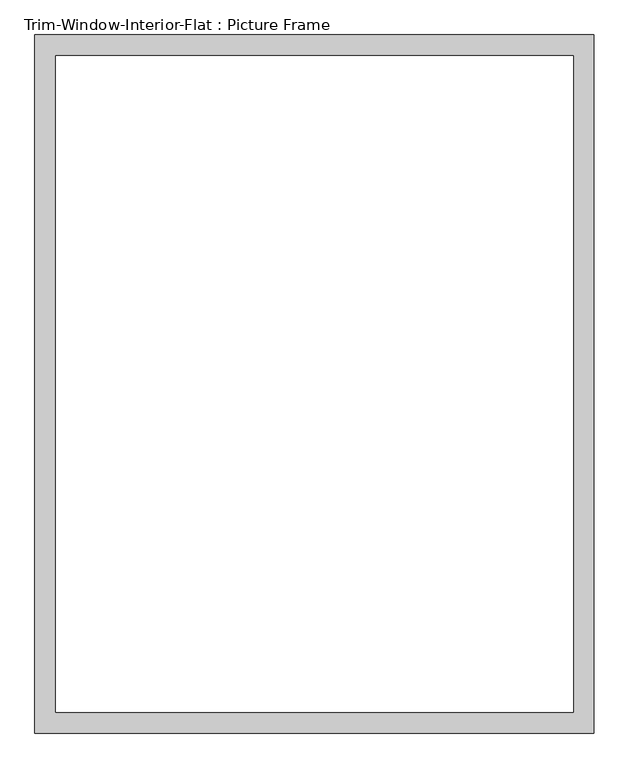
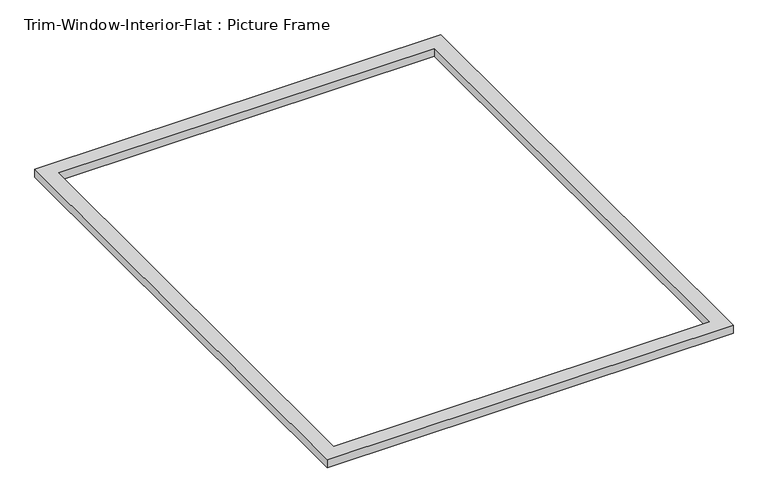
"""IFC4 building model written with IfcOpenShell, lengths in millimetres: proxy geometry, Trim-Window-Interior-Flat : Picture Frame."""

import ifcopenshell
import ifcopenshell.guid

model = None  # the IFC model being written
_history = None  # IfcOwnerHistory: only IFC2X3 demands one
_inside = {}  # id of a spatial element -> (the spatial element, [elements in it])
_under = {}  # id of a project, library or spatial element -> (it, [spatial elements below it])
_declared = {}  # id of a project -> (the project, [libraries it declares])
_typed = {}  # id of a type object -> (the type object, [elements of that type])
_made_of = {}  # id of a material, layer set ... -> (it, [elements and type objects made of it])


def new_model(schema):
    """Start an empty IFC model of exactly this schema.

    Asked for "IFC4X3", IfcOpenShell would pick the latest addendum, in which some entities
    have other attributes; the version numbers below select the first issue.
    IFC2X3 requires an IfcOwnerHistory on every rooted entity: one is made here for all.
    """
    global model, _history
    if schema == "IFC4X3":
        model = ifcopenshell.file(schema_version=(4, 3, 0, 0))
    else:
        model = ifcopenshell.file(schema=schema)
    _inside.clear()
    _under.clear()
    _declared.clear()
    _typed.clear()
    _made_of.clear()
    _history = None
    if model.schema == "IFC2X3":
        org = make("IfcOrganization", Name="unknown")
        user = make(
            "IfcPersonAndOrganization",
            ThePerson=make("IfcPerson", FamilyName="unknown"),
            TheOrganization=org,
        )
        app = make(
            "IfcApplication",
            ApplicationDeveloper=org,
            Version="unknown",
            ApplicationFullName="unknown",
            ApplicationIdentifier="unknown",
        )
        _history = make(
            "IfcOwnerHistory",
            OwningUser=user,
            OwningApplication=app,
            ChangeAction="ADDED",
            CreationDate=0,
        )
    return model


def make(cls, **values):
    """One entity of the class cls with the attributes given. An attribute that is None is left unset."""
    return model.create_entity(
        cls, **{name: value for name, value in values.items() if value is not None}
    )


def rooted(cls, **values):
    """An entity with a GlobalId (a new one), such as an element, a storey or a relation."""
    return make(cls, GlobalId=ifcopenshell.guid.new(), OwnerHistory=_history, **values)


def si_unit(unit_type, name, prefix=None):
    """IfcSIUnit, for example si_unit("LENGTHUNIT", "METRE", prefix="MILLI")."""
    return make("IfcSIUnit", UnitType=unit_type, Prefix=prefix, Name=name)


def assignment(units):
    """IfcUnitAssignment: the units of a project."""
    return None if units is None else make("IfcUnitAssignment", Units=units)


def point(xyz):
    """IfcCartesianPoint."""
    return None if xyz is None else make("IfcCartesianPoint", Coordinates=xyz)


def direction(xyz):
    """IfcDirection."""
    return None if xyz is None else make("IfcDirection", DirectionRatios=xyz)


def frame(location, z_axis=None, x_axis=None):
    """IfcAxis2Placement3D, a coordinate frame: its origin and axes. An axis left out is left unset."""
    return make(
        "IfcAxis2Placement3D",
        Location=point(location),
        Axis=direction(z_axis),
        RefDirection=direction(x_axis),
    )


def origin():
    """The frame at (0, 0, 0) with its axes left unset."""
    return frame((0.0, 0.0, 0.0))


def origin_with_axes():
    """The frame at (0, 0, 0) with the z axis (0, 0, 1) and the x axis (1, 0, 0) written out."""
    return frame((0.0, 0.0, 0.0), z_axis=(0.0, 0.0, 1.0), x_axis=(1.0, 0.0, 0.0))


def place(relative_to, where):
    """IfcLocalPlacement: puts the frame where relative to a parent placement (None: the world)."""
    return make(
        "IfcLocalPlacement", PlacementRelTo=relative_to, RelativePlacement=where
    )


def context(
    kind, dimensions, precision=None, world=None, true_north=None, identifier=None
):
    """IfcGeometricRepresentationContext, for example the 3D "Model" context."""
    return make(
        "IfcGeometricRepresentationContext",
        ContextIdentifier=identifier,
        ContextType=kind,
        CoordinateSpaceDimension=dimensions,
        Precision=precision,
        WorldCoordinateSystem=world,
        TrueNorth=true_north,
    )


def project(units=None, contexts=None):
    """IfcProject with its units and contexts."""
    return rooted(
        "IfcProject",
        Name="project",
        RepresentationContexts=contexts,
        UnitsInContext=assignment(units),
    )


def spatial(cls, under=None, at=None, **own):
    """A site, building, storey or space (cls), placed at a placement, below another one or the project."""
    s = rooted(cls, ObjectPlacement=at, **own)
    if under is not None:
        _under.setdefault(under.id(), (under, []))[1].append(s)
    return s


def polyline(points):
    """IfcPolyline through the points."""
    return make("IfcPolyline", Points=[point(p) for p in points])


def outline(outer, holes=None, kind="AREA"):
    """IfcArbitraryClosedProfileDef: a profile drawn as a closed curve; with holes, ...WithVoids."""
    if holes is None:
        return make("IfcArbitraryClosedProfileDef", ProfileType=kind, OuterCurve=outer)
    return make(
        "IfcArbitraryProfileDefWithVoids",
        ProfileType=kind,
        OuterCurve=outer,
        InnerCurves=holes,
    )


def extrude(swept, where, along, depth):
    """IfcExtrudedAreaSolid: the profile swept, set in the frame where, extruded along a direction by depth."""
    return make(
        "IfcExtrudedAreaSolid",
        SweptArea=swept,
        Position=where,
        ExtrudedDirection=direction(along),
        Depth=depth,
    )


def shape(context_of_items, identifier, shape_type, items):
    """IfcShapeRepresentation: the items that make up one representation, for example the "Body"."""
    return make(
        "IfcShapeRepresentation",
        ContextOfItems=context_of_items,
        RepresentationIdentifier=identifier,
        RepresentationType=shape_type,
        Items=items,
    )


def source(mapping_origin, context_of_items, identifier, shape_type, items):
    """IfcRepresentationMap: a shape defined once, which mapped items show again and again."""
    return make(
        "IfcRepresentationMap",
        MappingOrigin=mapping_origin,
        MappedRepresentation=shape(context_of_items, identifier, shape_type, items),
    )


def transform(
    local_origin,
    x_axis=None,
    y_axis=None,
    z_axis=None,
    scale=None,
    scale2=None,
    scale3=None,
    uniform=True,
):
    """IfcCartesianTransformationOperator3D, or its non-uniform kind. x_axis, y_axis, z_axis: its Axis1, 2, 3."""
    if uniform:
        return make(
            "IfcCartesianTransformationOperator3D",
            Axis1=direction(x_axis),
            Axis2=direction(y_axis),
            LocalOrigin=point(local_origin),
            Scale=scale,
            Axis3=direction(z_axis),
        )
    return make(
        "IfcCartesianTransformationOperator3DnonUniform",
        Axis1=direction(x_axis),
        Axis2=direction(y_axis),
        LocalOrigin=point(local_origin),
        Scale=scale,
        Axis3=direction(z_axis),
        Scale2=scale2,
        Scale3=scale3,
    )


def mapped(mapping_source, mapping_target):
    """IfcMappedItem: shows the shape of a source again, moved by a transform."""
    return make(
        "IfcMappedItem", MappingSource=mapping_source, MappingTarget=mapping_target
    )


def made_of(thing, what):
    """Note that an element or type object is made of a material, layer set ...; save() writes the relation."""
    if what is not None:
        _made_of.setdefault(what.id(), (what, []))[1].append(thing)
    return thing


def element(
    cls,
    number,
    at=None,
    inside=None,
    cuts=None,
    type_object=None,
    material=None,
    context=None,
    identifier="Body",
    shape_type=None,
    held_by="IfcProductDefinitionShape",
    body=None,
    shapes=None,
    **own,
):
    """One element of the class cls, such as IfcWall. Its Tag is "e" and its number.

    at: its placement. inside: the storey or other place that contains it. cuts: it is an
    opening in that element (IfcRelVoidsElement). A single representation is given by context,
    identifier, shape_type and body (its items); several are given by shapes. held_by: the class
    of the entity that holds the representations. save() writes the other relations.
    """
    e = rooted(cls, Tag="e%d" % number, ObjectPlacement=at, **own)
    if body is not None:
        shapes = [shape(context, identifier, shape_type, body)]
    if shapes is not None:
        e.Representation = make(held_by, Representations=shapes)
    if inside is not None:
        _inside.setdefault(inside.id(), (inside, []))[1].append(e)
    if cuts is not None:
        rooted(
            "IfcRelVoidsElement", RelatingBuildingElement=cuts, RelatedOpeningElement=e
        )
    if type_object is not None:
        _typed.setdefault(type_object.id(), (type_object, []))[1].append(e)
    return made_of(e, material)


def aggregate(whole, parts):
    """IfcRelAggregates: a whole, such as a stair, and the parts it consists of."""
    return rooted("IfcRelAggregates", RelatingObject=whole, RelatedObjects=parts)


def save(model, path):
    """Write the relations noted so far, then the file.

    IfcRelAggregates (storeys below a building ...), IfcRelContainedInSpatialStructure (elements
    in a storey), IfcRelDefinesByType, IfcRelAssociatesMaterial and IfcRelDeclares: one each for
    every whole, place, type object, material and project.
    """
    for whole, parts in _under.values():
        aggregate(whole, parts)
    for where, things in _inside.values():
        rooted(
            "IfcRelContainedInSpatialStructure",
            RelatedElements=things,
            RelatingStructure=where,
        )
    for kind, things in _typed.values():
        rooted("IfcRelDefinesByType", RelatedObjects=things, RelatingType=kind)
    for what, things in _made_of.values():
        rooted("IfcRelAssociatesMaterial", RelatedObjects=things, RelatingMaterial=what)
    for by, libraries in _declared.values():
        rooted("IfcRelDeclares", RelatingContext=by, RelatedDefinitions=libraries)
    model.write(path)


def trim_window_interior_flat_picture_frame_2a7685fe(model_context):
    return source(origin(), model_context, "Body", "SweptSolid", [
        extrude(outline(polyline([(768.35, 44.45), (768.35, -1873.25), (-768.35, -1873.25), (-768.35, 44.45), (768.35, 44.45)]), holes=[polyline([(711.2, -12.7), (-711.2, -12.7), (-711.2, -1816.1), (711.2, -1816.1), (711.2, -12.7)])]), origin_with_axes(), (0.0, 0.0, 1.0), 31.75),
    ])


if __name__ == "__main__":
    model = new_model("IFC4")
    model_context = context("Model", 3, world=origin())
    ifc_project = project(units=[si_unit("LENGTHUNIT", "METRE", prefix="MILLI")], contexts=[model_context])
    site = spatial("IfcSite", under=ifc_project)
    building = spatial("IfcBuilding", under=site)
    placement = place(None, origin())
    trim_window_interior_flat_picture_frame_shape = trim_window_interior_flat_picture_frame_2a7685fe(model_context)
    element("IfcBuildingElementProxy", 1, Name="Trim-Window-Interior-Flat : Picture Frame", ObjectType="Trim-Window-Interior-Flat : Picture Frame", at=placement, inside=building, context=model_context, shape_type="MappedRepresentation", body=[
        mapped(trim_window_interior_flat_picture_frame_shape, transform((0.0, 0.0, 0.0), x_axis=(1.0, 0.0, 0.0), y_axis=(0.0, 1.0, 0.0), z_axis=(0.0, 0.0, 1.0))),
    ])
    save(model, "model.ifc")

# Revit data of these elements
# Type "Trim-Window-Interior-Flat : Picture Frame"
#   Trim Thickness_Picture Frame = 0' - 1 1/4"
#   Trim Width = 0' - 2 1/4"
#   Trim Thickness_with Sill = 0' - 0 3/4"
#   Sill Thickness = 0' - 1 1/4"
#   Opening Width [instance default] = 2' - 0"
#   Opening Height [instance default] = 3' - 0"
#   Default Elevation = 4' - 0"
#   Sill = no
#   Picture Frame = yes
#   Trim Material [instance default] = none
# Element 1 (IfcBuildingElementProxy, "Trim-Window-Interior-Flat : Picture Frame")
#   Opening Width = 4' - 9"
#   Opening Height = 6' - 0"
#   Trim Material = Wood - Stained
#   Materials on its faces: "Wood - Stained"
# Materials
#   "Wood - Stained": class "Wood", colour RGB 224 178 126, transparency 0, Cost = 0
